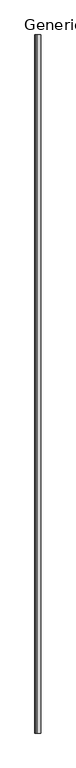
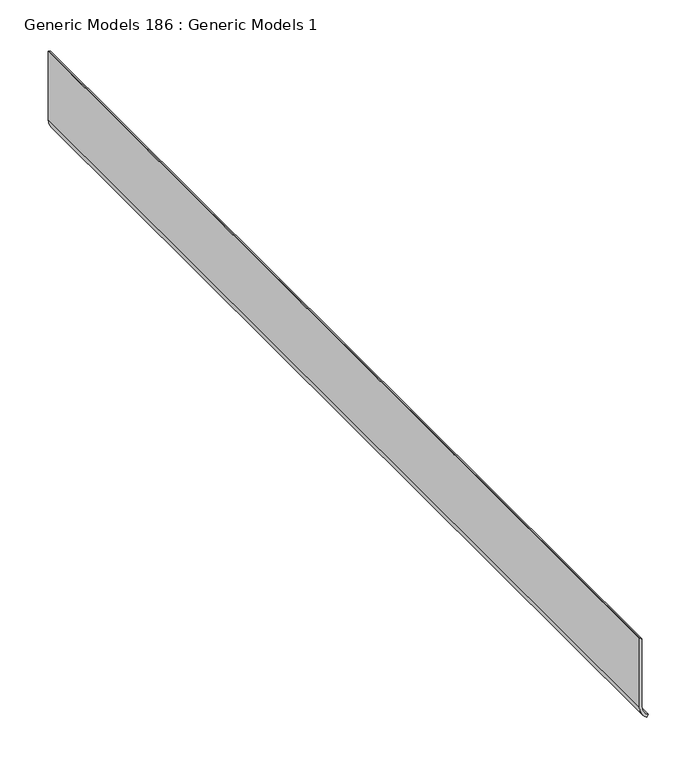
"""IFC4 building model written with IfcOpenShell, lengths in millimetres: proxy geometry, Generic Models 186 : Generic Models 1."""

import ifcopenshell
import ifcopenshell.guid

model = None  # the IFC model being written
_history = None  # IfcOwnerHistory: only IFC2X3 demands one
_inside = {}  # id of a spatial element -> (the spatial element, [elements in it])
_under = {}  # id of a project, library or spatial element -> (it, [spatial elements below it])
_declared = {}  # id of a project -> (the project, [libraries it declares])
_typed = {}  # id of a type object -> (the type object, [elements of that type])
_made_of = {}  # id of a material, layer set ... -> (it, [elements and type objects made of it])


def new_model(schema):
    """Start an empty IFC model of exactly this schema.

    Asked for "IFC4X3", IfcOpenShell would pick the latest addendum, in which some entities
    have other attributes; the version numbers below select the first issue.
    IFC2X3 requires an IfcOwnerHistory on every rooted entity: one is made here for all.
    """
    global model, _history
    if schema == "IFC4X3":
        model = ifcopenshell.file(schema_version=(4, 3, 0, 0))
    else:
        model = ifcopenshell.file(schema=schema)
    _inside.clear()
    _under.clear()
    _declared.clear()
    _typed.clear()
    _made_of.clear()
    _history = None
    if model.schema == "IFC2X3":
        org = make("IfcOrganization", Name="unknown")
        user = make(
            "IfcPersonAndOrganization",
            ThePerson=make("IfcPerson", FamilyName="unknown"),
            TheOrganization=org,
        )
        app = make(
            "IfcApplication",
            ApplicationDeveloper=org,
            Version="unknown",
            ApplicationFullName="unknown",
            ApplicationIdentifier="unknown",
        )
        _history = make(
            "IfcOwnerHistory",
            OwningUser=user,
            OwningApplication=app,
            ChangeAction="ADDED",
            CreationDate=0,
        )
    return model


def make(cls, **values):
    """One entity of the class cls with the attributes given. An attribute that is None is left unset."""
    return model.create_entity(
        cls, **{name: value for name, value in values.items() if value is not None}
    )


def rooted(cls, **values):
    """An entity with a GlobalId (a new one), such as an element, a storey or a relation."""
    return make(cls, GlobalId=ifcopenshell.guid.new(), OwnerHistory=_history, **values)


def si_unit(unit_type, name, prefix=None):
    """IfcSIUnit, for example si_unit("LENGTHUNIT", "METRE", prefix="MILLI")."""
    return make("IfcSIUnit", UnitType=unit_type, Prefix=prefix, Name=name)


def assignment(units):
    """IfcUnitAssignment: the units of a project."""
    return None if units is None else make("IfcUnitAssignment", Units=units)


def point(xyz):
    """IfcCartesianPoint."""
    return None if xyz is None else make("IfcCartesianPoint", Coordinates=xyz)


def direction(xyz):
    """IfcDirection."""
    return None if xyz is None else make("IfcDirection", DirectionRatios=xyz)


def frame(location, z_axis=None, x_axis=None):
    """IfcAxis2Placement3D, a coordinate frame: its origin and axes. An axis left out is left unset."""
    return make(
        "IfcAxis2Placement3D",
        Location=point(location),
        Axis=direction(z_axis),
        RefDirection=direction(x_axis),
    )


def frame_2d(location, x_axis=None):
    """IfcAxis2Placement2D, a coordinate frame in the plane: its origin and x axis."""
    return make(
        "IfcAxis2Placement2D", Location=point(location), RefDirection=direction(x_axis)
    )


def origin():
    """The frame at (0, 0, 0) with its axes left unset."""
    return frame((0.0, 0.0, 0.0))


def place(relative_to, where):
    """IfcLocalPlacement: puts the frame where relative to a parent placement (None: the world)."""
    return make(
        "IfcLocalPlacement", PlacementRelTo=relative_to, RelativePlacement=where
    )


def context(
    kind, dimensions, precision=None, world=None, true_north=None, identifier=None
):
    """IfcGeometricRepresentationContext, for example the 3D "Model" context."""
    return make(
        "IfcGeometricRepresentationContext",
        ContextIdentifier=identifier,
        ContextType=kind,
        CoordinateSpaceDimension=dimensions,
        Precision=precision,
        WorldCoordinateSystem=world,
        TrueNorth=true_north,
    )


def project(units=None, contexts=None):
    """IfcProject with its units and contexts."""
    return rooted(
        "IfcProject",
        Name="project",
        RepresentationContexts=contexts,
        UnitsInContext=assignment(units),
    )


def spatial(cls, under=None, at=None, **own):
    """A site, building, storey or space (cls), placed at a placement, below another one or the project."""
    s = rooted(cls, ObjectPlacement=at, **own)
    if under is not None:
        _under.setdefault(under.id(), (under, []))[1].append(s)
    return s


def polyline(points):
    """IfcPolyline through the points."""
    return make("IfcPolyline", Points=[point(p) for p in points])


def circle_curve(where, radius):
    """IfcCircle in the frame where."""
    return make("IfcCircle", Position=where, Radius=radius)


def trimmed(basis, trim1, trim2, sense, master):
    """IfcTrimmedCurve: the piece of a basis curve between two trims."""
    return make(
        "IfcTrimmedCurve",
        BasisCurve=basis,
        Trim1=trim1,
        Trim2=trim2,
        SenseAgreement=sense,
        MasterRepresentation=master,
    )


def segment(curve, same_sense, transition):
    """IfcCompositeCurveSegment."""
    return make(
        "IfcCompositeCurveSegment",
        Transition=transition,
        SameSense=same_sense,
        ParentCurve=curve,
    )


def composite_curve(segments, self_intersect=None):
    """IfcCompositeCurve: segments joined end to end."""
    return make("IfcCompositeCurve", Segments=segments, SelfIntersect=self_intersect)


def outline(outer, holes=None, kind="AREA"):
    """IfcArbitraryClosedProfileDef: a profile drawn as a closed curve; with holes, ...WithVoids."""
    if holes is None:
        return make("IfcArbitraryClosedProfileDef", ProfileType=kind, OuterCurve=outer)
    return make(
        "IfcArbitraryProfileDefWithVoids",
        ProfileType=kind,
        OuterCurve=outer,
        InnerCurves=holes,
    )


def extrude(swept, where, along, depth):
    """IfcExtrudedAreaSolid: the profile swept, set in the frame where, extruded along a direction by depth."""
    return make(
        "IfcExtrudedAreaSolid",
        SweptArea=swept,
        Position=where,
        ExtrudedDirection=direction(along),
        Depth=depth,
    )


def shape(context_of_items, identifier, shape_type, items):
    """IfcShapeRepresentation: the items that make up one representation, for example the "Body"."""
    return make(
        "IfcShapeRepresentation",
        ContextOfItems=context_of_items,
        RepresentationIdentifier=identifier,
        RepresentationType=shape_type,
        Items=items,
    )


def source(mapping_origin, context_of_items, identifier, shape_type, items):
    """IfcRepresentationMap: a shape defined once, which mapped items show again and again."""
    return make(
        "IfcRepresentationMap",
        MappingOrigin=mapping_origin,
        MappedRepresentation=shape(context_of_items, identifier, shape_type, items),
    )


def transform(
    local_origin,
    x_axis=None,
    y_axis=None,
    z_axis=None,
    scale=None,
    scale2=None,
    scale3=None,
    uniform=True,
):
    """IfcCartesianTransformationOperator3D, or its non-uniform kind. x_axis, y_axis, z_axis: its Axis1, 2, 3."""
    if uniform:
        return make(
            "IfcCartesianTransformationOperator3D",
            Axis1=direction(x_axis),
            Axis2=direction(y_axis),
            LocalOrigin=point(local_origin),
            Scale=scale,
            Axis3=direction(z_axis),
        )
    return make(
        "IfcCartesianTransformationOperator3DnonUniform",
        Axis1=direction(x_axis),
        Axis2=direction(y_axis),
        LocalOrigin=point(local_origin),
        Scale=scale,
        Axis3=direction(z_axis),
        Scale2=scale2,
        Scale3=scale3,
    )


def mapped(mapping_source, mapping_target):
    """IfcMappedItem: shows the shape of a source again, moved by a transform."""
    return make(
        "IfcMappedItem", MappingSource=mapping_source, MappingTarget=mapping_target
    )


def made_of(thing, what):
    """Note that an element or type object is made of a material, layer set ...; save() writes the relation."""
    if what is not None:
        _made_of.setdefault(what.id(), (what, []))[1].append(thing)
    return thing


def element(
    cls,
    number,
    at=None,
    inside=None,
    cuts=None,
    type_object=None,
    material=None,
    context=None,
    identifier="Body",
    shape_type=None,
    held_by="IfcProductDefinitionShape",
    body=None,
    shapes=None,
    **own,
):
    """One element of the class cls, such as IfcWall. Its Tag is "e" and its number.

    at: its placement. inside: the storey or other place that contains it. cuts: it is an
    opening in that element (IfcRelVoidsElement). A single representation is given by context,
    identifier, shape_type and body (its items); several are given by shapes. held_by: the class
    of the entity that holds the representations. save() writes the other relations.
    """
    e = rooted(cls, Tag="e%d" % number, ObjectPlacement=at, **own)
    if body is not None:
        shapes = [shape(context, identifier, shape_type, body)]
    if shapes is not None:
        e.Representation = make(held_by, Representations=shapes)
    if inside is not None:
        _inside.setdefault(inside.id(), (inside, []))[1].append(e)
    if cuts is not None:
        rooted(
            "IfcRelVoidsElement", RelatingBuildingElement=cuts, RelatedOpeningElement=e
        )
    if type_object is not None:
        _typed.setdefault(type_object.id(), (type_object, []))[1].append(e)
    return made_of(e, material)


def aggregate(whole, parts):
    """IfcRelAggregates: a whole, such as a stair, and the parts it consists of."""
    return rooted("IfcRelAggregates", RelatingObject=whole, RelatedObjects=parts)


def save(model, path):
    """Write the relations noted so far, then the file.

    IfcRelAggregates (storeys below a building ...), IfcRelContainedInSpatialStructure (elements
    in a storey), IfcRelDefinesByType, IfcRelAssociatesMaterial and IfcRelDeclares: one each for
    every whole, place, type object, material and project.
    """
    for whole, parts in _under.values():
        aggregate(whole, parts)
    for where, things in _inside.values():
        rooted(
            "IfcRelContainedInSpatialStructure",
            RelatedElements=things,
            RelatingStructure=where,
        )
    for kind, things in _typed.values():
        rooted("IfcRelDefinesByType", RelatedObjects=things, RelatingType=kind)
    for what, things in _made_of.values():
        rooted("IfcRelAssociatesMaterial", RelatedObjects=things, RelatingMaterial=what)
    for by, libraries in _declared.values():
        rooted("IfcRelDeclares", RelatingContext=by, RelatedDefinitions=libraries)
    model.write(path)


def generic_models_186_generic_models_1_f329077b(model_context):
    return source(origin(), model_context, "Body", "SweptSolid", [
        extrude(outline(composite_curve([segment(polyline([(-1822.8473206, 52666.3196108), (-1908.9976899, 52666.3196108)]), True, "CONTINUOUS"), segment(trimmed(circle_curve(frame_2d((-1908.9976899, 52684.1593077)), 17.8396968), [point((-1908.9976899, 52666.3196108))], [point((-1924.4473206, 52675.2394592))], False, "CARTESIAN"), True, "CONTINUOUS"), segment(polyline([(-1924.4473206, 52675.2394592), (-1921.6976899, 52676.8269592)]), True, "CONTINUOUS"), segment(trimmed(circle_curve(frame_2d((-1908.9976899, 52684.1593077)), 14.6646968), [point((-1921.6976899, 52676.8269592))], [point((-1908.9976899, 52669.4946108))], True, "CARTESIAN"), True, "CONTINUOUS"), segment(polyline([(-1908.9976899, 52669.4946108), (-1824.9341224, 52669.4946108)]), True, "CONTINUOUS"), segment(trimmed(circle_curve(frame_2d((-1824.9341224, 52667.407809)), 2.0868018), [point((-1824.9341224, 52669.4946108))], [point((-1822.8473206, 52667.407809))], False, "CARTESIAN"), True, "CONTINUOUS"), segment(polyline([(-1822.8473206, 52667.407809), (-1822.8473206, 52666.3196108)]), True, "CONTINUOUS")], self_intersect=False)), frame((0.0, 0.0, 0.0), z_axis=(0.0, 1.0, 0.0), x_axis=(0.0, 0.0, 1.0)), (0.0, 0.0, 1.0), 1219.2),
    ])


if __name__ == "__main__":
    model = new_model("IFC4")
    model_context = context("Model", 3, world=origin())
    ifc_project = project(units=[si_unit("LENGTHUNIT", "METRE", prefix="MILLI")], contexts=[model_context])
    site = spatial("IfcSite", under=ifc_project)
    building = spatial("IfcBuilding", under=site)
    placement = place(None, origin())
    generic_models_186_generic_models_1_shape = generic_models_186_generic_models_1_f329077b(model_context)
    element("IfcBuildingElementProxy", 1, Name="Generic Models 186 : Generic Models 1", ObjectType="Generic Models 186 : Generic Models 1", at=placement, inside=building, context=model_context, shape_type="MappedRepresentation", body=[
        mapped(generic_models_186_generic_models_1_shape, transform((0.0, 0.0, 0.0), x_axis=(1.0, 0.0, 0.0), y_axis=(0.0, 1.0, 0.0), z_axis=(0.0, 0.0, 1.0))),
    ])
    save(model, "model.ifc")

# Revit data of these elements
# Element 1 (IfcBuildingElementProxy, "Generic Models 186 : Generic Models 1")
#   Materials on its faces: "BASE T.B.D."
# Materials
#   "BASE T.B.D.": class "Generic", colour RGB 120 120 120, transparency 0, Cost = 0
